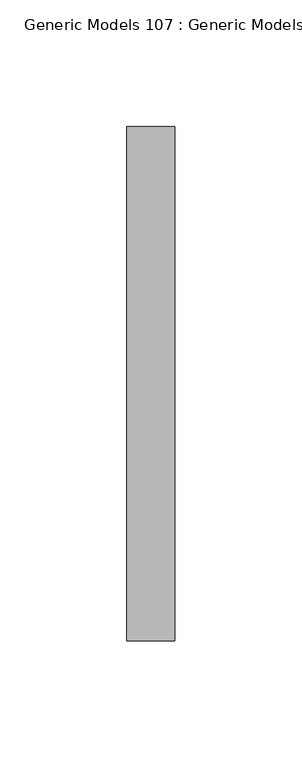
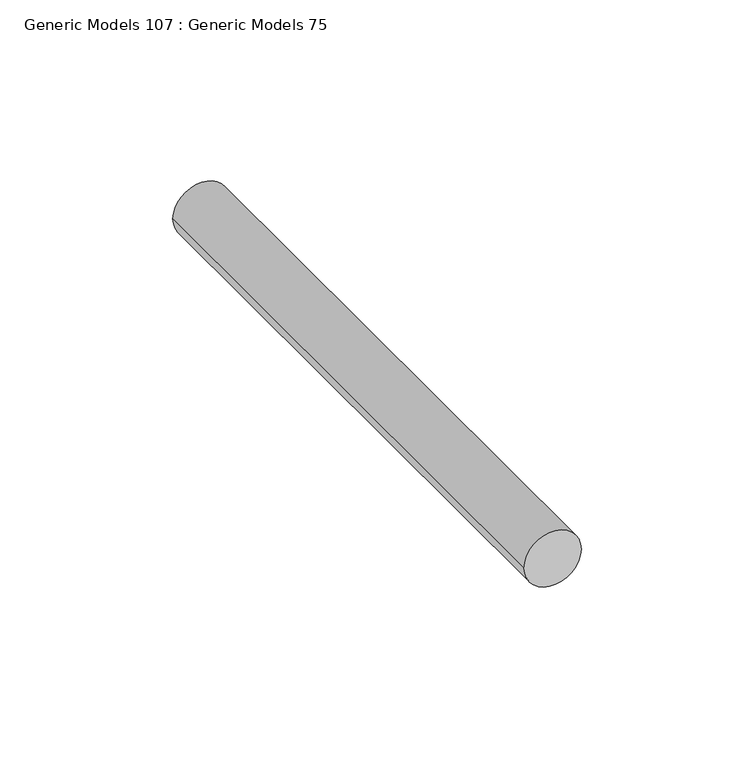
"""IFC4 building model written with IfcOpenShell, lengths in millimetres: proxy geometry, Generic Models 107 : Generic Models 75."""

from ifc_helpers import new_model, si_unit, point, frame, frame_2d, origin, place, context, project, spatial, circle_curve, trimmed, segment, composite_curve, outline, extrude, source, transform, mapped, element, save


def generic_models_107_generic_models_75_b10bc95d(model_context):
    return source(origin(), model_context, "Body", "SweptSolid", [
        extrude(outline(composite_curve([segment(trimmed(circle_curve(frame_2d((268495.4625, 31975.4096032)), 9.525), [point((268495.4625, 31965.8846032))], [point((268495.4625, 31984.9346032))], False, "CARTESIAN"), True, "CONTINUOUS"), segment(trimmed(circle_curve(frame_2d((268495.4625, 31975.4096032)), 9.525), [point((268495.4625, 31984.9346032))], [point((268495.4625, 31965.8846032))], False, "CARTESIAN"), True, "CONTINUOUS")], self_intersect=False)), frame((0.0, 30672.7406612, 0.0), z_axis=(0.0, 1.0, 0.0), x_axis=(0.0, 0.0, 1.0)), (0.0, 0.0, 1.0), 203.2),
    ])


if __name__ == "__main__":
    model = new_model("IFC4")
    model_context = context("Model", 3, world=origin())
    ifc_project = project(units=[si_unit("LENGTHUNIT", "METRE", prefix="MILLI")], contexts=[model_context])
    site = spatial("IfcSite", under=ifc_project)
    building = spatial("IfcBuilding", under=site)
    placement = place(None, origin())
    generic_models_107_generic_models_75_shape = generic_models_107_generic_models_75_b10bc95d(model_context)
    element("IfcBuildingElementProxy", 1, Name="Generic Models 107 : Generic Models 75", ObjectType="Generic Models 107 : Generic Models 75", at=placement, inside=building, context=model_context, shape_type="MappedRepresentation", body=[
        mapped(generic_models_107_generic_models_75_shape, transform((0.0, 0.0, 0.0), x_axis=(1.0, 0.0, 0.0), y_axis=(0.0, 1.0, 0.0), z_axis=(0.0, 0.0, 1.0))),
    ])
    save(model, "model.ifc")
